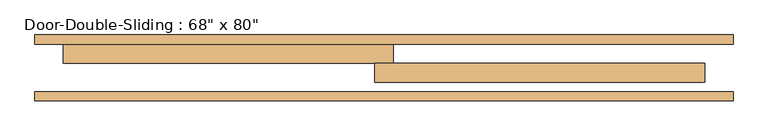
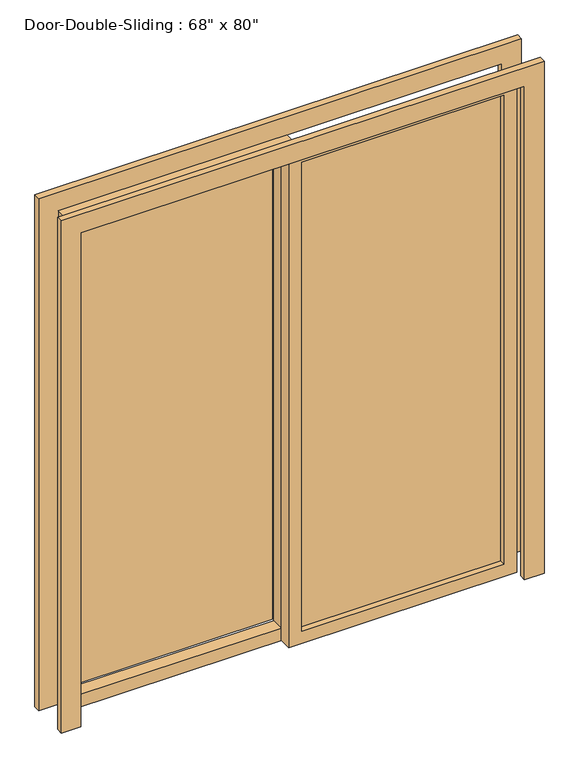
"""IFC4 building model written with IfcOpenShell, lengths in millimetres: door geometry."""

import ifcopenshell
import ifcopenshell.guid

model = None  # the IFC model being written
_history = None  # IfcOwnerHistory: only IFC2X3 demands one
_inside = {}  # id of a spatial element -> (the spatial element, [elements in it])
_under = {}  # id of a project, library or spatial element -> (it, [spatial elements below it])
_declared = {}  # id of a project -> (the project, [libraries it declares])
_typed = {}  # id of a type object -> (the type object, [elements of that type])
_made_of = {}  # id of a material, layer set ... -> (it, [elements and type objects made of it])


def new_model(schema):
    """Start an empty IFC model of exactly this schema.

    Asked for "IFC4X3", IfcOpenShell would pick the latest addendum, in which some entities
    have other attributes; the version numbers below select the first issue.
    IFC2X3 requires an IfcOwnerHistory on every rooted entity: one is made here for all.
    """
    global model, _history
    if schema == "IFC4X3":
        model = ifcopenshell.file(schema_version=(4, 3, 0, 0))
    else:
        model = ifcopenshell.file(schema=schema)
    _inside.clear()
    _under.clear()
    _declared.clear()
    _typed.clear()
    _made_of.clear()
    _history = None
    if model.schema == "IFC2X3":
        org = make("IfcOrganization", Name="unknown")
        user = make(
            "IfcPersonAndOrganization",
            ThePerson=make("IfcPerson", FamilyName="unknown"),
            TheOrganization=org,
        )
        app = make(
            "IfcApplication",
            ApplicationDeveloper=org,
            Version="unknown",
            ApplicationFullName="unknown",
            ApplicationIdentifier="unknown",
        )
        _history = make(
            "IfcOwnerHistory",
            OwningUser=user,
            OwningApplication=app,
            ChangeAction="ADDED",
            CreationDate=0,
        )
    return model


def make(cls, **values):
    """One entity of the class cls with the attributes given. An attribute that is None is left unset."""
    return model.create_entity(
        cls, **{name: value for name, value in values.items() if value is not None}
    )


def rooted(cls, **values):
    """An entity with a GlobalId (a new one), such as an element, a storey or a relation."""
    return make(cls, GlobalId=ifcopenshell.guid.new(), OwnerHistory=_history, **values)


def si_unit(unit_type, name, prefix=None):
    """IfcSIUnit, for example si_unit("LENGTHUNIT", "METRE", prefix="MILLI")."""
    return make("IfcSIUnit", UnitType=unit_type, Prefix=prefix, Name=name)


def assignment(units):
    """IfcUnitAssignment: the units of a project."""
    return None if units is None else make("IfcUnitAssignment", Units=units)


def point(xyz):
    """IfcCartesianPoint."""
    return None if xyz is None else make("IfcCartesianPoint", Coordinates=xyz)


def direction(xyz):
    """IfcDirection."""
    return None if xyz is None else make("IfcDirection", DirectionRatios=xyz)


def frame(location, z_axis=None, x_axis=None):
    """IfcAxis2Placement3D, a coordinate frame: its origin and axes. An axis left out is left unset."""
    return make(
        "IfcAxis2Placement3D",
        Location=point(location),
        Axis=direction(z_axis),
        RefDirection=direction(x_axis),
    )


def origin():
    """The frame at (0, 0, 0) with its axes left unset."""
    return frame((0.0, 0.0, 0.0))


def place(relative_to, where):
    """IfcLocalPlacement: puts the frame where relative to a parent placement (None: the world)."""
    return make(
        "IfcLocalPlacement", PlacementRelTo=relative_to, RelativePlacement=where
    )


def context(
    kind, dimensions, precision=None, world=None, true_north=None, identifier=None
):
    """IfcGeometricRepresentationContext, for example the 3D "Model" context."""
    return make(
        "IfcGeometricRepresentationContext",
        ContextIdentifier=identifier,
        ContextType=kind,
        CoordinateSpaceDimension=dimensions,
        Precision=precision,
        WorldCoordinateSystem=world,
        TrueNorth=true_north,
    )


def project(units=None, contexts=None):
    """IfcProject with its units and contexts."""
    return rooted(
        "IfcProject",
        Name="project",
        RepresentationContexts=contexts,
        UnitsInContext=assignment(units),
    )


def spatial(cls, under=None, at=None, **own):
    """A site, building, storey or space (cls), placed at a placement, below another one or the project."""
    s = rooted(cls, ObjectPlacement=at, **own)
    if under is not None:
        _under.setdefault(under.id(), (under, []))[1].append(s)
    return s


def polyline(points):
    """IfcPolyline through the points."""
    return make("IfcPolyline", Points=[point(p) for p in points])


def outline(outer, holes=None, kind="AREA"):
    """IfcArbitraryClosedProfileDef: a profile drawn as a closed curve; with holes, ...WithVoids."""
    if holes is None:
        return make("IfcArbitraryClosedProfileDef", ProfileType=kind, OuterCurve=outer)
    return make(
        "IfcArbitraryProfileDefWithVoids",
        ProfileType=kind,
        OuterCurve=outer,
        InnerCurves=holes,
    )


def extrude(swept, where, along, depth):
    """IfcExtrudedAreaSolid: the profile swept, set in the frame where, extruded along a direction by depth."""
    return make(
        "IfcExtrudedAreaSolid",
        SweptArea=swept,
        Position=where,
        ExtrudedDirection=direction(along),
        Depth=depth,
    )


def shape(context_of_items, identifier, shape_type, items):
    """IfcShapeRepresentation: the items that make up one representation, for example the "Body"."""
    return make(
        "IfcShapeRepresentation",
        ContextOfItems=context_of_items,
        RepresentationIdentifier=identifier,
        RepresentationType=shape_type,
        Items=items,
    )


def source(mapping_origin, context_of_items, identifier, shape_type, items):
    """IfcRepresentationMap: a shape defined once, which mapped items show again and again."""
    return make(
        "IfcRepresentationMap",
        MappingOrigin=mapping_origin,
        MappedRepresentation=shape(context_of_items, identifier, shape_type, items),
    )


def transform(
    local_origin,
    x_axis=None,
    y_axis=None,
    z_axis=None,
    scale=None,
    scale2=None,
    scale3=None,
    uniform=True,
):
    """IfcCartesianTransformationOperator3D, or its non-uniform kind. x_axis, y_axis, z_axis: its Axis1, 2, 3."""
    if uniform:
        return make(
            "IfcCartesianTransformationOperator3D",
            Axis1=direction(x_axis),
            Axis2=direction(y_axis),
            LocalOrigin=point(local_origin),
            Scale=scale,
            Axis3=direction(z_axis),
        )
    return make(
        "IfcCartesianTransformationOperator3DnonUniform",
        Axis1=direction(x_axis),
        Axis2=direction(y_axis),
        LocalOrigin=point(local_origin),
        Scale=scale,
        Axis3=direction(z_axis),
        Scale2=scale2,
        Scale3=scale3,
    )


def mapped(mapping_source, mapping_target):
    """IfcMappedItem: shows the shape of a source again, moved by a transform."""
    return make(
        "IfcMappedItem", MappingSource=mapping_source, MappingTarget=mapping_target
    )


def made_of(thing, what):
    """Note that an element or type object is made of a material, layer set ...; save() writes the relation."""
    if what is not None:
        _made_of.setdefault(what.id(), (what, []))[1].append(thing)
    return thing


def element(
    cls,
    number,
    at=None,
    inside=None,
    cuts=None,
    type_object=None,
    material=None,
    context=None,
    identifier="Body",
    shape_type=None,
    held_by="IfcProductDefinitionShape",
    body=None,
    shapes=None,
    **own,
):
    """One element of the class cls, such as IfcWall. Its Tag is "e" and its number.

    at: its placement. inside: the storey or other place that contains it. cuts: it is an
    opening in that element (IfcRelVoidsElement). A single representation is given by context,
    identifier, shape_type and body (its items); several are given by shapes. held_by: the class
    of the entity that holds the representations. save() writes the other relations.
    """
    e = rooted(cls, Tag="e%d" % number, ObjectPlacement=at, **own)
    if body is not None:
        shapes = [shape(context, identifier, shape_type, body)]
    if shapes is not None:
        e.Representation = make(held_by, Representations=shapes)
    if inside is not None:
        _inside.setdefault(inside.id(), (inside, []))[1].append(e)
    if cuts is not None:
        rooted(
            "IfcRelVoidsElement", RelatingBuildingElement=cuts, RelatedOpeningElement=e
        )
    if type_object is not None:
        _typed.setdefault(type_object.id(), (type_object, []))[1].append(e)
    return made_of(e, material)


def aggregate(whole, parts):
    """IfcRelAggregates: a whole, such as a stair, and the parts it consists of."""
    return rooted("IfcRelAggregates", RelatingObject=whole, RelatedObjects=parts)


def save(model, path):
    """Write the relations noted so far, then the file.

    IfcRelAggregates (storeys below a building ...), IfcRelContainedInSpatialStructure (elements
    in a storey), IfcRelDefinesByType, IfcRelAssociatesMaterial and IfcRelDeclares: one each for
    every whole, place, type object, material and project.
    """
    for whole, parts in _under.values():
        aggregate(whole, parts)
    for where, things in _inside.values():
        rooted(
            "IfcRelContainedInSpatialStructure",
            RelatedElements=things,
            RelatingStructure=where,
        )
    for kind, things in _typed.values():
        rooted("IfcRelDefinesByType", RelatedObjects=things, RelatingType=kind)
    for what, things in _made_of.values():
        rooted("IfcRelAssociatesMaterial", RelatedObjects=things, RelatingMaterial=what)
    for by, libraries in _declared.values():
        rooted("IfcRelDeclares", RelatingContext=by, RelatedDefinitions=libraries)
    model.write(path)


def door_87897aa2(model_context):
    return source(origin(), model_context, "Body", "SweptSolid", [
        extrude(outline(polyline([(0.0, -939.8), (0.0, -863.6), (2032.0, -863.6), (2032.0, 863.6), (0.0, 863.6), (0.0, 939.8), (2108.2, 939.8), (2108.2, -939.8), (0.0, -939.8)])), frame((0.0, 38.1, 0.0), z_axis=(0.0, 1.0, 0.0), x_axis=(0.0, 0.0, 1.0)), (0.0, 0.0, 1.0), 25.4),
        extrude(outline(polyline([(0.0, 939.8), (2108.2, 939.8), (2108.2, -939.8), (0.0, -939.8), (0.0, -863.6), (2032.0, -863.6), (2032.0, 863.6), (0.0, 863.6), (0.0, 939.8)])), frame((0.0, 190.5, 0.0), z_axis=(0.0, 1.0, 0.0), x_axis=(0.0, 0.0, 1.0)), (0.0, 0.0, 1.0), 25.4),
        extrude(outline(polyline([(2032.0, -25.4), (0.0, -25.4), (0.0, 863.6), (2032.0, 863.6), (2032.0, -25.4)]), holes=[polyline([(1981.2, 25.4), (1981.2, 812.8), (50.8, 812.8), (50.8, 25.4), (1981.2, 25.4)])]), frame((0.0, 88.9, 0.0), z_axis=(0.0, 1.0, 0.0), x_axis=(0.0, 0.0, 1.0)), (0.0, 0.0, 1.0), 50.8),
        extrude(outline(polyline([(2032.0, 25.4), (2032.0, -863.6), (0.0, -863.6), (0.0, 25.4), (2032.0, 25.4)]), holes=[polyline([(1981.2, -25.4), (50.8, -25.4), (50.8, -812.8), (1981.2, -812.8), (1981.2, -25.4)])]), frame((0.0, 139.7, 0.0), z_axis=(0.0, 1.0, 0.0), x_axis=(0.0, 0.0, 1.0)), (0.0, 0.0, 1.0), 50.8),
        extrude(outline(polyline([(25.4, 117.475), (812.8, 117.475), (812.8, 111.125), (25.4, 111.125), (25.4, 117.475)])), frame((0.0, 0.0, 50.8), z_axis=(0.0, 0.0, 1.0), x_axis=(1.0, 0.0, 0.0)), (0.0, 0.0, 1.0), 1930.4),
        extrude(outline(polyline([(-25.4, 200.025), (-812.8, 200.025), (-812.8, 206.375), (-25.4, 206.375), (-25.4, 200.025)])), frame((0.0, 0.0, 50.8), z_axis=(0.0, 0.0, 1.0), x_axis=(1.0, 0.0, 0.0)), (0.0, 0.0, 1.0), 1930.4),
    ])


if __name__ == "__main__":
    model = new_model("IFC4")
    model_context = context("Model", 3, world=origin())
    ifc_project = project(units=[si_unit("LENGTHUNIT", "METRE", prefix="MILLI")], contexts=[model_context])
    site = spatial("IfcSite", under=ifc_project)
    building = spatial("IfcBuilding", under=site)
    placement = place(None, origin())
    door_shape = door_87897aa2(model_context)
    element("IfcDoor", 1, ObjectType="Door-Double-Sliding : 68\" x 80\"", at=placement, inside=building, context=model_context, shape_type="MappedRepresentation", body=[
        mapped(door_shape, transform((0.0, 0.0, 0.0), x_axis=(1.0, 0.0, 0.0), y_axis=(0.0, 1.0, 0.0), z_axis=(0.0, 0.0, 1.0))),
    ])
    save(model, "model.ifc")

# Revit data of these elements
# Type "Door-Double-Sliding : 68\" x 80\""
#   Type Mark = "8"
#   Construction Type Id = "opn-d45"
#   Assembly Code = "C1020"
#   Analytic Construction = "Wood frame, double glass door "
#   Thickness = 0.0508 m
#   Thermal Resistance (R) = 0.31964 (m²·K)/W
#   Heat Transfer Coefficient (U) = 3.12872 W/(m²·K)
#   Height = 2.032 m
#   Rail Width = 0.0508 m
#   Stiles = 0.0508 m
#   Trim Projection Ext = 0.0254 m
#   Trim Projection Int = 0.0254 m
#   Trim Width = 0.0762 m
#   Width = 1.7272 m
#   Glazing = Glass
#   Panel Material = Wood - Birch - Solid Stained Light Low Gloss
#   Trim Material = Paint - Sienna
#   Visual Light Transmittance = 0
#   Solar Heat Gain Coefficient = 0
#   Function = (empty or 0)
#   Wall Closure = (empty or 0)
# Element 1 (IfcDoor, "Door-Double-Sliding : 68\" x 80\"")
#   Materials on its faces: "Paint - Sienna", "Wood - Birch - Solid Stained Light Low Gloss", "Glass"
# Materials
#   "Glass": class "Glass", colour RGB 213 204 197, transparency 0.85, Description = "Soda Lime Glass", Cost = 0
#   "Wood - Birch - Solid Stained Light Low Gloss": class "Wood", colour RGB 227 170 128, transparency 0, Cost = 0
#   "Paint - Sienna": class "Miscellaneous", colour RGB 118 70 51, transparency 0, Cost = 0
